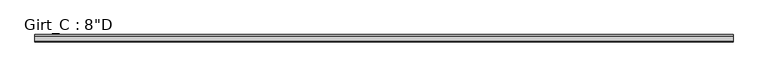
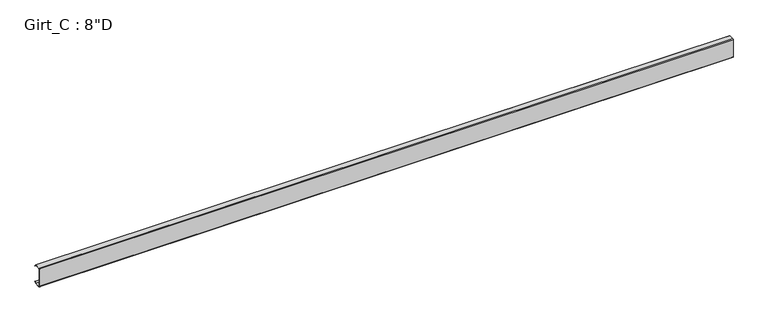
"""IFC4 building model written with IfcOpenShell, lengths in millimetres: beam geometry."""

import ifcopenshell
import ifcopenshell.guid

model = None  # the IFC model being written
_history = None  # IfcOwnerHistory: only IFC2X3 demands one
_inside = {}  # id of a spatial element -> (the spatial element, [elements in it])
_under = {}  # id of a project, library or spatial element -> (it, [spatial elements below it])
_declared = {}  # id of a project -> (the project, [libraries it declares])
_typed = {}  # id of a type object -> (the type object, [elements of that type])
_made_of = {}  # id of a material, layer set ... -> (it, [elements and type objects made of it])


def new_model(schema):
    """Start an empty IFC model of exactly this schema.

    Asked for "IFC4X3", IfcOpenShell would pick the latest addendum, in which some entities
    have other attributes; the version numbers below select the first issue.
    IFC2X3 requires an IfcOwnerHistory on every rooted entity: one is made here for all.
    """
    global model, _history
    if schema == "IFC4X3":
        model = ifcopenshell.file(schema_version=(4, 3, 0, 0))
    else:
        model = ifcopenshell.file(schema=schema)
    _inside.clear()
    _under.clear()
    _declared.clear()
    _typed.clear()
    _made_of.clear()
    _history = None
    if model.schema == "IFC2X3":
        org = make("IfcOrganization", Name="unknown")
        user = make(
            "IfcPersonAndOrganization",
            ThePerson=make("IfcPerson", FamilyName="unknown"),
            TheOrganization=org,
        )
        app = make(
            "IfcApplication",
            ApplicationDeveloper=org,
            Version="unknown",
            ApplicationFullName="unknown",
            ApplicationIdentifier="unknown",
        )
        _history = make(
            "IfcOwnerHistory",
            OwningUser=user,
            OwningApplication=app,
            ChangeAction="ADDED",
            CreationDate=0,
        )
    return model


def make(cls, **values):
    """One entity of the class cls with the attributes given. An attribute that is None is left unset."""
    return model.create_entity(
        cls, **{name: value for name, value in values.items() if value is not None}
    )


def rooted(cls, **values):
    """An entity with a GlobalId (a new one), such as an element, a storey or a relation."""
    return make(cls, GlobalId=ifcopenshell.guid.new(), OwnerHistory=_history, **values)


def si_unit(unit_type, name, prefix=None):
    """IfcSIUnit, for example si_unit("LENGTHUNIT", "METRE", prefix="MILLI")."""
    return make("IfcSIUnit", UnitType=unit_type, Prefix=prefix, Name=name)


def assignment(units):
    """IfcUnitAssignment: the units of a project."""
    return None if units is None else make("IfcUnitAssignment", Units=units)


def point(xyz):
    """IfcCartesianPoint."""
    return None if xyz is None else make("IfcCartesianPoint", Coordinates=xyz)


def direction(xyz):
    """IfcDirection."""
    return None if xyz is None else make("IfcDirection", DirectionRatios=xyz)


def frame(location, z_axis=None, x_axis=None):
    """IfcAxis2Placement3D, a coordinate frame: its origin and axes. An axis left out is left unset."""
    return make(
        "IfcAxis2Placement3D",
        Location=point(location),
        Axis=direction(z_axis),
        RefDirection=direction(x_axis),
    )


def frame_2d(location, x_axis=None):
    """IfcAxis2Placement2D, a coordinate frame in the plane: its origin and x axis."""
    return make(
        "IfcAxis2Placement2D", Location=point(location), RefDirection=direction(x_axis)
    )


def origin():
    """The frame at (0, 0, 0) with its axes left unset."""
    return frame((0.0, 0.0, 0.0))


def place(relative_to, where):
    """IfcLocalPlacement: puts the frame where relative to a parent placement (None: the world)."""
    return make(
        "IfcLocalPlacement", PlacementRelTo=relative_to, RelativePlacement=where
    )


def context(
    kind, dimensions, precision=None, world=None, true_north=None, identifier=None
):
    """IfcGeometricRepresentationContext, for example the 3D "Model" context."""
    return make(
        "IfcGeometricRepresentationContext",
        ContextIdentifier=identifier,
        ContextType=kind,
        CoordinateSpaceDimension=dimensions,
        Precision=precision,
        WorldCoordinateSystem=world,
        TrueNorth=true_north,
    )


def project(units=None, contexts=None):
    """IfcProject with its units and contexts."""
    return rooted(
        "IfcProject",
        Name="project",
        RepresentationContexts=contexts,
        UnitsInContext=assignment(units),
    )


def spatial(cls, under=None, at=None, **own):
    """A site, building, storey or space (cls), placed at a placement, below another one or the project."""
    s = rooted(cls, ObjectPlacement=at, **own)
    if under is not None:
        _under.setdefault(under.id(), (under, []))[1].append(s)
    return s


def polyline(points):
    """IfcPolyline through the points."""
    return make("IfcPolyline", Points=[point(p) for p in points])


def circle_curve(where, radius):
    """IfcCircle in the frame where."""
    return make("IfcCircle", Position=where, Radius=radius)


def trimmed(basis, trim1, trim2, sense, master):
    """IfcTrimmedCurve: the piece of a basis curve between two trims."""
    return make(
        "IfcTrimmedCurve",
        BasisCurve=basis,
        Trim1=trim1,
        Trim2=trim2,
        SenseAgreement=sense,
        MasterRepresentation=master,
    )


def segment(curve, same_sense, transition):
    """IfcCompositeCurveSegment."""
    return make(
        "IfcCompositeCurveSegment",
        Transition=transition,
        SameSense=same_sense,
        ParentCurve=curve,
    )


def composite_curve(segments, self_intersect=None):
    """IfcCompositeCurve: segments joined end to end."""
    return make("IfcCompositeCurve", Segments=segments, SelfIntersect=self_intersect)


def outline(outer, holes=None, kind="AREA"):
    """IfcArbitraryClosedProfileDef: a profile drawn as a closed curve; with holes, ...WithVoids."""
    if holes is None:
        return make("IfcArbitraryClosedProfileDef", ProfileType=kind, OuterCurve=outer)
    return make(
        "IfcArbitraryProfileDefWithVoids",
        ProfileType=kind,
        OuterCurve=outer,
        InnerCurves=holes,
    )


def extrude(swept, where, along, depth):
    """IfcExtrudedAreaSolid: the profile swept, set in the frame where, extruded along a direction by depth."""
    return make(
        "IfcExtrudedAreaSolid",
        SweptArea=swept,
        Position=where,
        ExtrudedDirection=direction(along),
        Depth=depth,
    )


def shape(context_of_items, identifier, shape_type, items):
    """IfcShapeRepresentation: the items that make up one representation, for example the "Body"."""
    return make(
        "IfcShapeRepresentation",
        ContextOfItems=context_of_items,
        RepresentationIdentifier=identifier,
        RepresentationType=shape_type,
        Items=items,
    )


def source(mapping_origin, context_of_items, identifier, shape_type, items):
    """IfcRepresentationMap: a shape defined once, which mapped items show again and again."""
    return make(
        "IfcRepresentationMap",
        MappingOrigin=mapping_origin,
        MappedRepresentation=shape(context_of_items, identifier, shape_type, items),
    )


def transform(
    local_origin,
    x_axis=None,
    y_axis=None,
    z_axis=None,
    scale=None,
    scale2=None,
    scale3=None,
    uniform=True,
):
    """IfcCartesianTransformationOperator3D, or its non-uniform kind. x_axis, y_axis, z_axis: its Axis1, 2, 3."""
    if uniform:
        return make(
            "IfcCartesianTransformationOperator3D",
            Axis1=direction(x_axis),
            Axis2=direction(y_axis),
            LocalOrigin=point(local_origin),
            Scale=scale,
            Axis3=direction(z_axis),
        )
    return make(
        "IfcCartesianTransformationOperator3DnonUniform",
        Axis1=direction(x_axis),
        Axis2=direction(y_axis),
        LocalOrigin=point(local_origin),
        Scale=scale,
        Axis3=direction(z_axis),
        Scale2=scale2,
        Scale3=scale3,
    )


def mapped(mapping_source, mapping_target):
    """IfcMappedItem: shows the shape of a source again, moved by a transform."""
    return make(
        "IfcMappedItem", MappingSource=mapping_source, MappingTarget=mapping_target
    )


def made_of(thing, what):
    """Note that an element or type object is made of a material, layer set ...; save() writes the relation."""
    if what is not None:
        _made_of.setdefault(what.id(), (what, []))[1].append(thing)
    return thing


def element(
    cls,
    number,
    at=None,
    inside=None,
    cuts=None,
    type_object=None,
    material=None,
    context=None,
    identifier="Body",
    shape_type=None,
    held_by="IfcProductDefinitionShape",
    body=None,
    shapes=None,
    **own,
):
    """One element of the class cls, such as IfcWall. Its Tag is "e" and its number.

    at: its placement. inside: the storey or other place that contains it. cuts: it is an
    opening in that element (IfcRelVoidsElement). A single representation is given by context,
    identifier, shape_type and body (its items); several are given by shapes. held_by: the class
    of the entity that holds the representations. save() writes the other relations.
    """
    e = rooted(cls, Tag="e%d" % number, ObjectPlacement=at, **own)
    if body is not None:
        shapes = [shape(context, identifier, shape_type, body)]
    if shapes is not None:
        e.Representation = make(held_by, Representations=shapes)
    if inside is not None:
        _inside.setdefault(inside.id(), (inside, []))[1].append(e)
    if cuts is not None:
        rooted(
            "IfcRelVoidsElement", RelatingBuildingElement=cuts, RelatedOpeningElement=e
        )
    if type_object is not None:
        _typed.setdefault(type_object.id(), (type_object, []))[1].append(e)
    return made_of(e, material)


def aggregate(whole, parts):
    """IfcRelAggregates: a whole, such as a stair, and the parts it consists of."""
    return rooted("IfcRelAggregates", RelatingObject=whole, RelatedObjects=parts)


def save(model, path):
    """Write the relations noted so far, then the file.

    IfcRelAggregates (storeys below a building ...), IfcRelContainedInSpatialStructure (elements
    in a storey), IfcRelDefinesByType, IfcRelAssociatesMaterial and IfcRelDeclares: one each for
    every whole, place, type object, material and project.
    """
    for whole, parts in _under.values():
        aggregate(whole, parts)
    for where, things in _inside.values():
        rooted(
            "IfcRelContainedInSpatialStructure",
            RelatedElements=things,
            RelatingStructure=where,
        )
    for kind, things in _typed.values():
        rooted("IfcRelDefinesByType", RelatedObjects=things, RelatingType=kind)
    for what, things in _made_of.values():
        rooted("IfcRelAssociatesMaterial", RelatedObjects=things, RelatingMaterial=what)
    for by, libraries in _declared.values():
        rooted("IfcRelDeclares", RelatingContext=by, RelatedDefinitions=libraries)
    model.write(path)


def beam_fcef19db(model_context):
    return source(origin(), model_context, "Body", "SweptSolid", [
        extrude(outline(composite_curve([segment(polyline([(63.5, 101.6), (75.745104, 87.0068534), (73.6169367, 85.221109), (62.204539, 98.821875), (3.3005807, 98.821875)]), True, "CONTINUOUS"), segment(trimmed(circle_curve(frame_2d((3.3741066, 96.8381931)), 1.9850441), [point((3.3005807, 98.821875))], [point((1.3890625, 96.8381931))], True, "CARTESIAN"), True, "CONTINUOUS"), segment(polyline([(1.3890625, 96.8381931), (1.3890625, -96.8389339)]), True, "CONTINUOUS"), segment(trimmed(circle_curve(frame_2d((3.3748024, -96.8389339)), 1.9857399), [point((1.3890625, -96.8389339))], [point((3.2694106, -98.821875))], True, "CARTESIAN"), True, "CONTINUOUS"), segment(polyline([(3.2694106, -98.821875), (62.204539, -98.821875), (73.6169367, -85.221109), (75.745104, -87.0068534), (63.5, -101.6), (3.3734375, -101.6)]), True, "CONTINUOUS"), segment(trimmed(circle_curve(frame_2d((3.3734375, -96.8375)), 4.7625), [point((3.3734375, -101.6))], [point((-1.3890625, -96.8375))], False, "CARTESIAN"), True, "CONTINUOUS"), segment(polyline([(-1.3890625, -96.8375), (-1.3890625, 96.8375)]), True, "CONTINUOUS"), segment(trimmed(circle_curve(frame_2d((3.3734375, 96.8375)), 4.7625), [point((-1.3890625, 96.8375))], [point((3.3734375, 101.6))], False, "CARTESIAN"), True, "CONTINUOUS"), segment(polyline([(3.3734375, 101.6), (63.5, 101.6)]), True, "CONTINUOUS")], self_intersect=False)), frame((-3623.3257261, 0.0, 0.0), z_axis=(1.0, 0.0, 0.0), x_axis=(0.0, 1.0, 0.0)), (0.0, 0.0, 1.0), 7251.7),
    ])


if __name__ == "__main__":
    model = new_model("IFC4")
    model_context = context("Model", 3, world=origin())
    ifc_project = project(units=[si_unit("LENGTHUNIT", "METRE", prefix="MILLI")], contexts=[model_context])
    site = spatial("IfcSite", under=ifc_project)
    building = spatial("IfcBuilding", under=site)
    placement = place(None, origin())
    beam_shape = beam_fcef19db(model_context)
    element("IfcBeam", 1, ObjectType="Girt_C : 8\"D", at=placement, inside=building, context=model_context, shape_type="MappedRepresentation", body=[
        mapped(beam_shape, transform((0.0, 0.0, 0.0), x_axis=(1.0, 0.0, 0.0), y_axis=(0.0, 1.0, 0.0), z_axis=(0.0, 0.0, 1.0))),
    ])
    save(model, "model.ifc")

# Revit data of these elements
# Type "Girt_C : 8\"D"
#   Web_Thickness = 0' - 0 7/64"
#   Length [instance default] = 10' - 0"
#   Leg_1 = 0' - 2 1/2"
#   Height = 0' - 8"
#   Structural Material [instance default] = none
# Element 1 (IfcBeam, "Girt_C : 8\"D")
#   Structural Material = Steel
#   Materials on its faces: "Steel"
# Materials
#   "Steel": class "Metal", colour RGB 118 118 114, transparency 0, Description = "Steel, mill finish", Cost = 0
